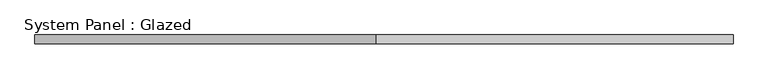
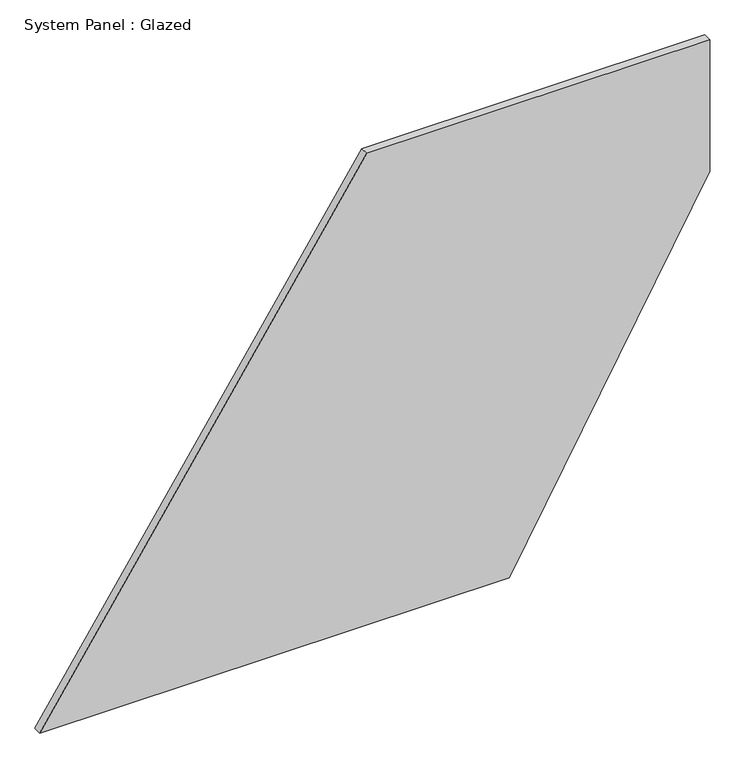
"""IFC4 building model written with IfcOpenShell, lengths in millimetres: plate geometry, System Panel : Glazed."""

import ifcopenshell
import ifcopenshell.guid

model = None  # the IFC model being written
_history = None  # IfcOwnerHistory: only IFC2X3 demands one
_inside = {}  # id of a spatial element -> (the spatial element, [elements in it])
_under = {}  # id of a project, library or spatial element -> (it, [spatial elements below it])
_declared = {}  # id of a project -> (the project, [libraries it declares])
_typed = {}  # id of a type object -> (the type object, [elements of that type])
_made_of = {}  # id of a material, layer set ... -> (it, [elements and type objects made of it])


def new_model(schema):
    """Start an empty IFC model of exactly this schema.

    Asked for "IFC4X3", IfcOpenShell would pick the latest addendum, in which some entities
    have other attributes; the version numbers below select the first issue.
    IFC2X3 requires an IfcOwnerHistory on every rooted entity: one is made here for all.
    """
    global model, _history
    if schema == "IFC4X3":
        model = ifcopenshell.file(schema_version=(4, 3, 0, 0))
    else:
        model = ifcopenshell.file(schema=schema)
    _inside.clear()
    _under.clear()
    _declared.clear()
    _typed.clear()
    _made_of.clear()
    _history = None
    if model.schema == "IFC2X3":
        org = make("IfcOrganization", Name="unknown")
        user = make(
            "IfcPersonAndOrganization",
            ThePerson=make("IfcPerson", FamilyName="unknown"),
            TheOrganization=org,
        )
        app = make(
            "IfcApplication",
            ApplicationDeveloper=org,
            Version="unknown",
            ApplicationFullName="unknown",
            ApplicationIdentifier="unknown",
        )
        _history = make(
            "IfcOwnerHistory",
            OwningUser=user,
            OwningApplication=app,
            ChangeAction="ADDED",
            CreationDate=0,
        )
    return model


def make(cls, **values):
    """One entity of the class cls with the attributes given. An attribute that is None is left unset."""
    return model.create_entity(
        cls, **{name: value for name, value in values.items() if value is not None}
    )


def rooted(cls, **values):
    """An entity with a GlobalId (a new one), such as an element, a storey or a relation."""
    return make(cls, GlobalId=ifcopenshell.guid.new(), OwnerHistory=_history, **values)


def si_unit(unit_type, name, prefix=None):
    """IfcSIUnit, for example si_unit("LENGTHUNIT", "METRE", prefix="MILLI")."""
    return make("IfcSIUnit", UnitType=unit_type, Prefix=prefix, Name=name)


def assignment(units):
    """IfcUnitAssignment: the units of a project."""
    return None if units is None else make("IfcUnitAssignment", Units=units)


def point(xyz):
    """IfcCartesianPoint."""
    return None if xyz is None else make("IfcCartesianPoint", Coordinates=xyz)


def direction(xyz):
    """IfcDirection."""
    return None if xyz is None else make("IfcDirection", DirectionRatios=xyz)


def frame(location, z_axis=None, x_axis=None):
    """IfcAxis2Placement3D, a coordinate frame: its origin and axes. An axis left out is left unset."""
    return make(
        "IfcAxis2Placement3D",
        Location=point(location),
        Axis=direction(z_axis),
        RefDirection=direction(x_axis),
    )


def origin():
    """The frame at (0, 0, 0) with its axes left unset."""
    return frame((0.0, 0.0, 0.0))


def place(relative_to, where):
    """IfcLocalPlacement: puts the frame where relative to a parent placement (None: the world)."""
    return make(
        "IfcLocalPlacement", PlacementRelTo=relative_to, RelativePlacement=where
    )


def context(
    kind, dimensions, precision=None, world=None, true_north=None, identifier=None
):
    """IfcGeometricRepresentationContext, for example the 3D "Model" context."""
    return make(
        "IfcGeometricRepresentationContext",
        ContextIdentifier=identifier,
        ContextType=kind,
        CoordinateSpaceDimension=dimensions,
        Precision=precision,
        WorldCoordinateSystem=world,
        TrueNorth=true_north,
    )


def project(units=None, contexts=None):
    """IfcProject with its units and contexts."""
    return rooted(
        "IfcProject",
        Name="project",
        RepresentationContexts=contexts,
        UnitsInContext=assignment(units),
    )


def spatial(cls, under=None, at=None, **own):
    """A site, building, storey or space (cls), placed at a placement, below another one or the project."""
    s = rooted(cls, ObjectPlacement=at, **own)
    if under is not None:
        _under.setdefault(under.id(), (under, []))[1].append(s)
    return s


def polyline(points):
    """IfcPolyline through the points."""
    return make("IfcPolyline", Points=[point(p) for p in points])


def outline(outer, holes=None, kind="AREA"):
    """IfcArbitraryClosedProfileDef: a profile drawn as a closed curve; with holes, ...WithVoids."""
    if holes is None:
        return make("IfcArbitraryClosedProfileDef", ProfileType=kind, OuterCurve=outer)
    return make(
        "IfcArbitraryProfileDefWithVoids",
        ProfileType=kind,
        OuterCurve=outer,
        InnerCurves=holes,
    )


def extrude(swept, where, along, depth):
    """IfcExtrudedAreaSolid: the profile swept, set in the frame where, extruded along a direction by depth."""
    return make(
        "IfcExtrudedAreaSolid",
        SweptArea=swept,
        Position=where,
        ExtrudedDirection=direction(along),
        Depth=depth,
    )


def shape(context_of_items, identifier, shape_type, items):
    """IfcShapeRepresentation: the items that make up one representation, for example the "Body"."""
    return make(
        "IfcShapeRepresentation",
        ContextOfItems=context_of_items,
        RepresentationIdentifier=identifier,
        RepresentationType=shape_type,
        Items=items,
    )


def source(mapping_origin, context_of_items, identifier, shape_type, items):
    """IfcRepresentationMap: a shape defined once, which mapped items show again and again."""
    return make(
        "IfcRepresentationMap",
        MappingOrigin=mapping_origin,
        MappedRepresentation=shape(context_of_items, identifier, shape_type, items),
    )


def transform(
    local_origin,
    x_axis=None,
    y_axis=None,
    z_axis=None,
    scale=None,
    scale2=None,
    scale3=None,
    uniform=True,
):
    """IfcCartesianTransformationOperator3D, or its non-uniform kind. x_axis, y_axis, z_axis: its Axis1, 2, 3."""
    if uniform:
        return make(
            "IfcCartesianTransformationOperator3D",
            Axis1=direction(x_axis),
            Axis2=direction(y_axis),
            LocalOrigin=point(local_origin),
            Scale=scale,
            Axis3=direction(z_axis),
        )
    return make(
        "IfcCartesianTransformationOperator3DnonUniform",
        Axis1=direction(x_axis),
        Axis2=direction(y_axis),
        LocalOrigin=point(local_origin),
        Scale=scale,
        Axis3=direction(z_axis),
        Scale2=scale2,
        Scale3=scale3,
    )


def mapped(mapping_source, mapping_target):
    """IfcMappedItem: shows the shape of a source again, moved by a transform."""
    return make(
        "IfcMappedItem", MappingSource=mapping_source, MappingTarget=mapping_target
    )


def made_of(thing, what):
    """Note that an element or type object is made of a material, layer set ...; save() writes the relation."""
    if what is not None:
        _made_of.setdefault(what.id(), (what, []))[1].append(thing)
    return thing


def element(
    cls,
    number,
    at=None,
    inside=None,
    cuts=None,
    type_object=None,
    material=None,
    context=None,
    identifier="Body",
    shape_type=None,
    held_by="IfcProductDefinitionShape",
    body=None,
    shapes=None,
    **own,
):
    """One element of the class cls, such as IfcWall. Its Tag is "e" and its number.

    at: its placement. inside: the storey or other place that contains it. cuts: it is an
    opening in that element (IfcRelVoidsElement). A single representation is given by context,
    identifier, shape_type and body (its items); several are given by shapes. held_by: the class
    of the entity that holds the representations. save() writes the other relations.
    """
    e = rooted(cls, Tag="e%d" % number, ObjectPlacement=at, **own)
    if body is not None:
        shapes = [shape(context, identifier, shape_type, body)]
    if shapes is not None:
        e.Representation = make(held_by, Representations=shapes)
    if inside is not None:
        _inside.setdefault(inside.id(), (inside, []))[1].append(e)
    if cuts is not None:
        rooted(
            "IfcRelVoidsElement", RelatingBuildingElement=cuts, RelatedOpeningElement=e
        )
    if type_object is not None:
        _typed.setdefault(type_object.id(), (type_object, []))[1].append(e)
    return made_of(e, material)


def aggregate(whole, parts):
    """IfcRelAggregates: a whole, such as a stair, and the parts it consists of."""
    return rooted("IfcRelAggregates", RelatingObject=whole, RelatedObjects=parts)


def save(model, path):
    """Write the relations noted so far, then the file.

    IfcRelAggregates (storeys below a building ...), IfcRelContainedInSpatialStructure (elements
    in a storey), IfcRelDefinesByType, IfcRelAssociatesMaterial and IfcRelDeclares: one each for
    every whole, place, type object, material and project.
    """
    for whole, parts in _under.values():
        aggregate(whole, parts)
    for where, things in _inside.values():
        rooted(
            "IfcRelContainedInSpatialStructure",
            RelatedElements=things,
            RelatingStructure=where,
        )
    for kind, things in _typed.values():
        rooted("IfcRelDefinesByType", RelatedObjects=things, RelatingType=kind)
    for what, things in _made_of.values():
        rooted("IfcRelAssociatesMaterial", RelatedObjects=things, RelatingMaterial=what)
    for by, libraries in _declared.values():
        rooted("IfcRelDeclares", RelatingContext=by, RelatedDefinitions=libraries)
    model.write(path)


def system_panel_glazed_a8889685(model_context):
    return source(origin(), model_context, "Body", "SweptSolid", [
        extrude(outline(polyline([(0.0, -1008.1540457), (0.0, 405.2562184), (1081.9101827, 1008.1540457), (1500.0, 1008.1540457), (1500.0, -24.4621368), (0.0, -1008.1540457)])), frame((0.0, 24.5, 0.0), z_axis=(0.0, 1.0, 0.0), x_axis=(0.0, 0.0, 1.0)), (0.0, 0.0, 1.0), 25.0),
    ])


if __name__ == "__main__":
    model = new_model("IFC4")
    model_context = context("Model", 3, world=origin())
    ifc_project = project(units=[si_unit("LENGTHUNIT", "METRE", prefix="MILLI")], contexts=[model_context])
    site = spatial("IfcSite", under=ifc_project)
    building = spatial("IfcBuilding", under=site)
    placement = place(None, origin())
    system_panel_glazed_shape = system_panel_glazed_a8889685(model_context)
    element("IfcPlate", 1, ObjectType="System Panel : Glazed", at=placement, inside=building, context=model_context, shape_type="MappedRepresentation", body=[
        mapped(system_panel_glazed_shape, transform((0.0, 0.0, 0.0), x_axis=(1.0, 0.0, 0.0), y_axis=(0.0, 1.0, 0.0), z_axis=(0.0, 0.0, 1.0))),
    ])
    save(model, "model.ifc")

# Revit data of these elements
# Type "System Panel : Glazed"
#   Construction Type Id = "GSP4R"
#   Analytic Construction = "1/8 in Pilkington single glazing"
#   Visual Light Transmittance = 0.9
#   Solar Heat Gain Coefficient = 0.86
#   Heat Transfer Coefficient (U) = 6.7069 W/(m²·K)
#   Define Thermal Properties by = 1
# Element 1 (IfcPlate, "System Panel : Glazed")
#   Materials on its faces: "Glass"
# Materials
#   "Glass": class "Glass", colour RGB 0 128 192, transparency 0.9, Description = "Soda Lime Glass", Cost = 0
